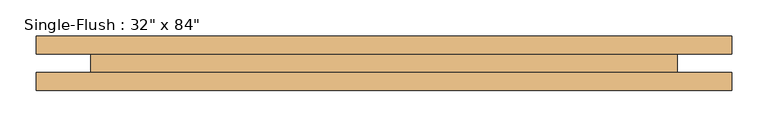
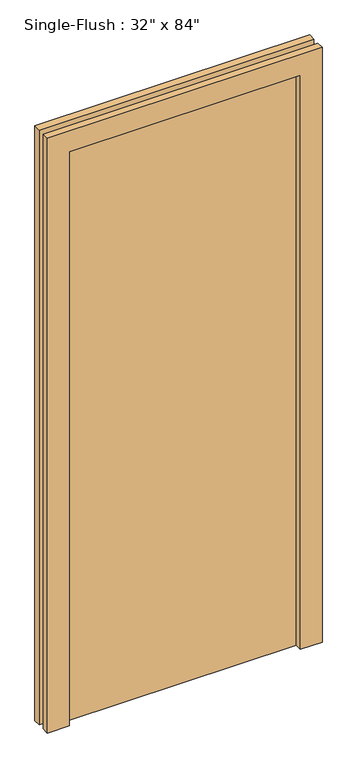
"""IFC4 building model written with IfcOpenShell, lengths in millimetres: door geometry."""

from ifc_helpers import new_model, si_unit, frame, origin, origin_with_axes, place, context, project, spatial, polyline, outline, extrude, source, transform, mapped, element, save


def door_5c1b3ce9(model_context):
    return source(origin(), model_context, "Body", "SweptSolid", [
        extrude(outline(polyline([(2209.8, -482.6), (0.0, -482.6), (0.0, -406.4), (2133.6, -406.4), (2133.6, 406.4), (0.0, 406.4), (0.0, 482.6), (2209.8, 482.6), (2209.8, -482.6)])), frame((0.0, -38.1, 0.0), z_axis=(0.0, 1.0, 0.0), x_axis=(0.0, 0.0, 1.0)), (0.0, 0.0, 1.0), 25.4),
        extrude(outline(polyline([(2209.8, 482.6), (2209.8, -482.6), (0.0, -482.6), (0.0, -406.4), (2133.6, -406.4), (2133.6, 406.4), (0.0, 406.4), (0.0, 482.6), (2209.8, 482.6)])), frame((0.0, 12.7, 0.0), z_axis=(0.0, 1.0, 0.0), x_axis=(0.0, 0.0, 1.0)), (0.0, 0.0, 1.0), 25.4),
        extrude(outline(polyline([(406.4, 38.1), (406.4, -12.7), (-406.4, -12.7), (-406.4, 38.1), (406.4, 38.1)])), origin_with_axes(), (0.0, 0.0, 1.0), 2133.6),
    ])


if __name__ == "__main__":
    model = new_model("IFC4")
    model_context = context("Model", 3, world=origin())
    ifc_project = project(units=[si_unit("LENGTHUNIT", "METRE", prefix="MILLI")], contexts=[model_context])
    site = spatial("IfcSite", under=ifc_project)
    building = spatial("IfcBuilding", under=site)
    placement = place(None, origin())
    door_shape = door_5c1b3ce9(model_context)
    element("IfcDoor", 1, ObjectType="Single-Flush : 32\" x 84\"", at=placement, inside=building, context=model_context, shape_type="MappedRepresentation", body=[
        mapped(door_shape, transform((0.0, 0.0, 0.0), x_axis=(1.0, 0.0, 0.0), y_axis=(0.0, 1.0, 0.0), z_axis=(0.0, 0.0, 1.0))),
    ])
    save(model, "model.ifc")

# Revit data of these elements
# Type "Single-Flush : 32\" x 84\""
#   Type Mark = "10"
#   Construction Type Id = "MDOOR"
#   Assembly Code = "C1020"
#   Analytic Construction = "Metal"
#   Thickness = 0' - 2"
#   Heat Transfer Coefficient (U) = 3.7021 W/(m²·K)
#   Height = 7' - 0"
#   Trim Projection Ext = 0' - 1"
#   Trim Projection Int = 0' - 1"
#   Trim Width = 0' - 3"
#   Width = 2' - 8"
#   Door Material = Door - Panel
#   Frame Material = Door - Frame
#   Visual Light Transmittance = 0
#   Solar Heat Gain Coefficient = 0
#   Function = (empty or 0)
#   Wall Closure = (empty or 0)
# Element 1 (IfcDoor, "Single-Flush : 32\" x 84\"")
#   Materials on its faces: "Door - Frame", "Door - Panel"
# Materials
#   "Door - Panel": class "Wood", colour RGB 210 159 95, transparency 0
#   "Door - Frame": class "Miscellaneous", colour RGB 118 70 51, transparency 0
